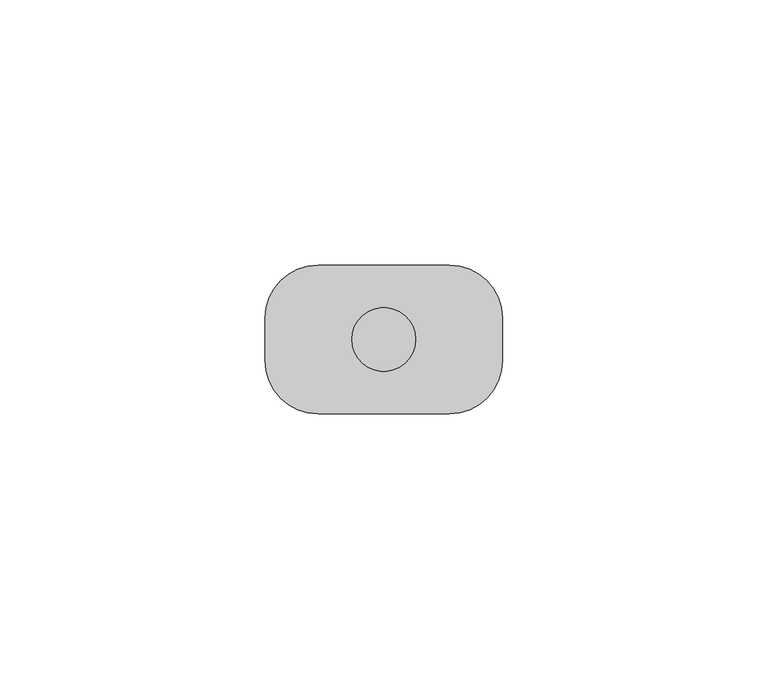
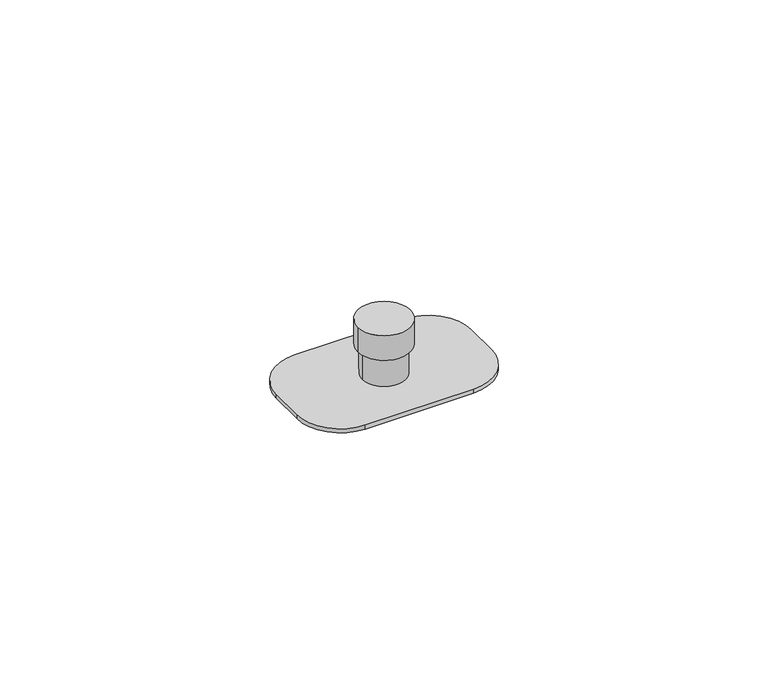
"""IFC4 building model written with IfcOpenShell, lengths in millimetres: proxy geometry, 12 mm Diameter Roller Wheel Sliding Wood Door Bottom Guide : 12 mm Diameter Roller Wheel Sliding Wood Door Bottom Guide."""

from ifc_helpers import new_model, si_unit, point, frame, frame_2d, origin, origin_with_axes, place, context, project, spatial, polyline, circle_curve, trimmed, segment, composite_curve, outline, extrude, source, transform, mapped, element, save


def generic_models_31eeb36d(model_context):
    return source(origin(), model_context, "Body", "SweptSolid", [
        extrude(outline(composite_curve([segment(trimmed(circle_curve(frame_2d((0.0, 0.3941037)), 6.0151312), [point((-6.0151312, 0.3941037))], [point((6.0151312, 0.3941037))], False, "CARTESIAN"), True, "CONTINUOUS"), segment(trimmed(circle_curve(frame_2d((0.0, 0.3941037)), 6.0151312), [point((6.0151312, 0.3941037))], [point((-6.0151312, 0.3941037))], False, "CARTESIAN"), True, "CONTINUOUS")], self_intersect=False)), frame((0.0, 0.0, 8.0), z_axis=(0.0, 0.0, 1.0), x_axis=(1.0, 0.0, 0.0)), (0.0, 0.0, 1.0), 6.0),
        extrude(outline(composite_curve([segment(trimmed(circle_curve(frame_2d((0.0, 0.3941037)), 5.0), [point((-5.0, 0.3941037))], [point((5.0, 0.3941037))], False, "CARTESIAN"), True, "CONTINUOUS"), segment(trimmed(circle_curve(frame_2d((0.0, 0.3941037)), 5.0), [point((5.0, 0.3941037))], [point((-5.0, 0.3941037))], False, "CARTESIAN"), True, "CONTINUOUS")], self_intersect=False)), frame((0.0, 0.0, 1.0), z_axis=(0.0, 0.0, 1.0), x_axis=(1.0, 0.0, 0.0)), (0.0, 0.0, 1.0), 7.0),
        extrude(outline(composite_curve([segment(polyline([(12.4077768, -13.6058963), (-12.4077768, -13.6058963)]), True, "CONTINUOUS"), segment(trimmed(circle_curve(frame_2d((-12.4077768, -3.6058963)), 10.0), [point((-12.4077768, -13.6058963))], [point((-22.4077768, -3.6058963))], False, "CARTESIAN"), True, "CONTINUOUS"), segment(polyline([(-22.4077768, -3.6058963), (-22.4077768, 4.3941037)]), True, "CONTINUOUS"), segment(trimmed(circle_curve(frame_2d((-12.4077768, 4.3941037)), 10.0), [point((-22.4077768, 4.3941037))], [point((-12.4077768, 14.3941037))], False, "CARTESIAN"), True, "CONTINUOUS"), segment(polyline([(-12.4077768, 14.3941037), (12.4077768, 14.3941037)]), True, "CONTINUOUS"), segment(trimmed(circle_curve(frame_2d((12.4077768, 4.3941037)), 10.0), [point((12.4077768, 14.3941037))], [point((22.4077768, 4.3941037))], False, "CARTESIAN"), True, "CONTINUOUS"), segment(polyline([(22.4077768, 4.3941037), (22.4077768, -3.6058963)]), True, "CONTINUOUS"), segment(trimmed(circle_curve(frame_2d((12.4077768, -3.6058963)), 10.0), [point((22.4077768, -3.6058963))], [point((12.4077768, -13.6058963))], False, "CARTESIAN"), True, "CONTINUOUS")], self_intersect=False)), origin_with_axes(), (0.0, 0.0, 1.0), 1.0),
    ])


if __name__ == "__main__":
    model = new_model("IFC4")
    model_context = context("Model", 3, world=origin())
    ifc_project = project(units=[si_unit("LENGTHUNIT", "METRE", prefix="MILLI")], contexts=[model_context])
    site = spatial("IfcSite", under=ifc_project)
    building = spatial("IfcBuilding", under=site)
    placement = place(None, origin())
    generic_models_shape = generic_models_31eeb36d(model_context)
    element("IfcBuildingElementProxy", 1, Name="12 mm Diameter Roller Wheel Sliding Wood Door Bottom Guide : 12 mm Diameter Roller Wheel Sliding Wood Door Bottom Guide", ObjectType="12 mm Diameter Roller Wheel Sliding Wood Door Bottom Guide : 12 mm Diameter Roller Wheel Sliding Wood Door Bottom Guide", at=placement, inside=building, context=model_context, shape_type="MappedRepresentation", body=[
        mapped(generic_models_shape, transform((0.0, 0.0, 0.0), x_axis=(1.0, 0.0, 0.0), y_axis=(0.0, 1.0, 0.0), z_axis=(0.0, 0.0, 1.0))),
    ])
    save(model, "model.ifc")

# Revit data of these elements
# Element 1 (IfcBuildingElementProxy, "12 mm Diameter Roller Wheel Sliding Wood Door Bottom Guide : 12 mm Diameter Roller Wheel Sliding Wood Door Bottom Guide")
#   Materials on its faces: "metal", "12 mm DIA. ROLLER WHEEL SLIDING WOOD DOOR BOTTOM GUIDE"
# Materials
#   "metal": class "Miscellaneous", colour RGB 127 127 127, transparency 0, Cost = 0
#   "12 mm DIA. ROLLER WHEEL SLIDING WOOD DOOR BOTTOM GUIDE": class "System", colour RGB 64 0 0, transparency 0, Cost = 0
